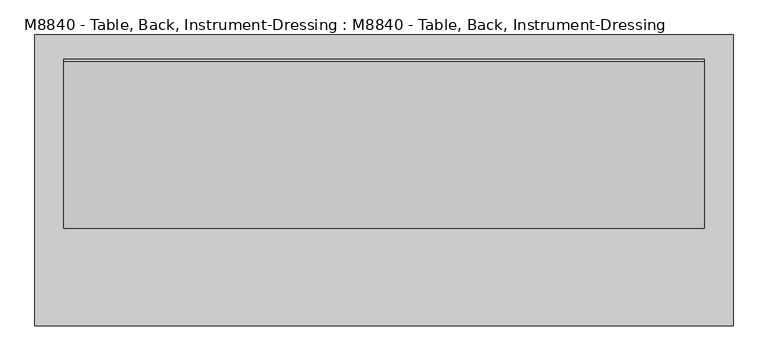
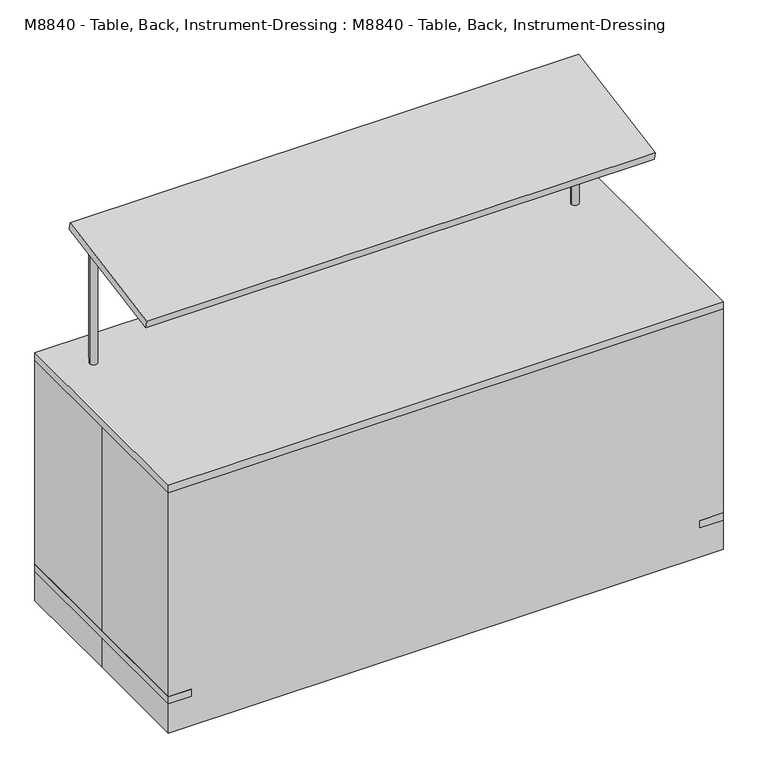
"""IFC4 building model written with IfcOpenShell, lengths in millimetres: proxy geometry, M8840 - Table, Back, Instrument-Dressing : M8840 - Table, Back, Instrument-Dressing."""

from ifc_helpers import new_model, si_unit, point, frame, frame_2d, origin, origin_with_axes, place, context, project, spatial, polyline, circle_curve, ellipse_curve, trimmed, segment, composite_curve, outline, extrude, source, transform, mapped, element, save
from ifc_brep_helpers import plane_surface, cylinder_surface, advanced_brep


def m8840_table_back_instrument_dressing_m8840_table_back_7214e6ad(model_context):
    return source(origin(), model_context, "Body", "SolidModel", [
        advanced_brep(
        [(838.2, 312.4393375, 1331.1669319), (-838.2, 312.4393375, 1331.1669319), (-838.2, -125.5940422, 1253.9298286), (838.2, -125.5940422, 1253.9298286), (838.2, 316.8500012, 1306.1528149), (838.2, -121.1833785, 1228.9157117), (-838.2, -121.1833785, 1228.9157117), (-838.2, 316.8500012, 1306.1528149), (-806.45, 255.8677573, 1295.4), (-781.05, 255.8677573, 1295.4), (806.45, 255.8677573, 1295.4), (781.05, 255.8677573, 1295.4), (-806.45, 255.8677573, 863.6), (-781.05, 255.8677573, 863.6), (806.45, 255.8677573, 863.6), (781.05, 255.8677573, 863.6)],
        [
            (0, 1),
            (1, 2),
            (2, 3),
            (3, 0),
            (4, 5),
            (5, 6),
            (6, 7),
            (7, 4),
            (8, 9, ellipse_curve(frame((-793.75, 255.8677573, 1295.4), z_axis=(0.0, -0.17364817766692925, 0.9848077530122082), x_axis=(0.0, 0.9848077530122081, 0.17364817766692942)), 12.895918, 12.7)),
            (9, 8, ellipse_curve(frame((-793.75, 255.8677573, 1295.4), z_axis=(0.0, -0.17364817766692925, 0.9848077530122082), x_axis=(0.0, 0.9848077530122081, 0.17364817766692942)), 12.895918, 12.7)),
            (10, 11, ellipse_curve(frame((793.75, 255.8677573, 1295.4), z_axis=(0.0, -0.17364817766692925, 0.9848077530122082), x_axis=(0.0, 0.9848077530122081, 0.17364817766692942)), 12.895918, 12.7)),
            (11, 10, ellipse_curve(frame((793.75, 255.8677573, 1295.4), z_axis=(0.0, -0.17364817766692925, 0.9848077530122082), x_axis=(0.0, 0.9848077530122081, 0.17364817766692942)), 12.895918, 12.7)),
            (0, 4),
            (7, 1),
            (6, 2),
            (5, 3),
            (12, 13, circle_curve(frame((-793.75, 255.8677573, 863.6), z_axis=(0.0, 0.0, -1.0), x_axis=(1.0, 0.0, 0.0)), 12.7)),
            (13, 12, circle_curve(frame((-793.75, 255.8677573, 863.6), z_axis=(0.0, 0.0, -1.0), x_axis=(1.0, 0.0, 0.0)), 12.7)),
            (14, 15, circle_curve(frame((793.75, 255.8677573, 863.6), z_axis=(0.0, 0.0, -1.0), x_axis=(-1.0, 0.0, 0.0)), 12.7)),
            (15, 14, circle_curve(frame((793.75, 255.8677573, 863.6), z_axis=(0.0, 0.0, -1.0), x_axis=(-1.0, 0.0, 0.0)), 12.7)),
            (13, 9),
            (8, 12),
            (15, 11),
            (10, 14),
        ],
        [
            plane_surface(frame((-838.2, 312.4393375, 1331.1669319), z_axis=(0.0, -0.17364817766692925, 0.9848077530122082), x_axis=(-1.0, 0.0, 0.0))),
            plane_surface(frame((-838.2, 316.8500012, 1306.1528149), z_axis=(0.0, 0.17364817766692925, -0.9848077530122082), x_axis=(1.0, 0.0, 0.0))),
            plane_surface(frame((838.2, 312.4393375, 1331.1669319), z_axis=(0.0, 0.9848077530122084, 0.17364817766692864), x_axis=(0.0, 0.17364817766692864, -0.9848077530122084))),
            plane_surface(frame((-838.2, 312.4393375, 1331.1669319), z_axis=(-1.0, 0.0, 0.0), x_axis=(0.0, 0.17364817766692864, -0.9848077530122084))),
            plane_surface(frame((-838.2, -125.5940422, 1253.9298286), z_axis=(0.0, -0.9848077530122079, -0.17364817766693125), x_axis=(0.0, 0.17364817766693125, -0.9848077530122079))),
            plane_surface(frame((838.2, -125.5940422, 1253.9298286), z_axis=(1.0, 0.0, 0.0), x_axis=(0.0, 0.17364817766692864, -0.9848077530122084))),
            plane_surface(frame((-781.05, 255.8677573, 863.6), z_axis=(0.0, 0.0, -1.0), x_axis=(0.0, -1.0, 0.0))),
            cylinder_surface(frame((-793.75, 255.8677573, 863.6), z_axis=(0.0, 0.0, 1.0), x_axis=(1.0, 0.0, 0.0)), 12.7),
            cylinder_surface(frame((793.75, 255.8677573, 0.0), z_axis=(0.0, 0.0, 1.0), x_axis=(-1.0, 0.0, 0.0)), 12.7),
        ],
        [
            (0, [[1, 2, 3, 4]]),
            (1, [[5, 6, 7, 8], [9, 10], [11, 12]]),
            (2, [[-1, 13, -8, 14]]),
            (3, [[-2, -14, -7, 15]]),
            (4, [[-3, -15, -6, 16]]),
            (5, [[-4, -16, -5, -13]]),
            (6, [[17, 18]]),
            (6, [[19, 20]]),
            (7, [[-18, 21, -9, 22]]),
            (7, [[-17, -22, -10, -21]]),
            (8, [[-20, 23, -11, 24]]),
            (8, [[-19, -24, -12, -23]]),
        ],
    ),
        extrude(outline(polyline([(869.95, 290.561646), (863.6, 290.561646), (863.6, 317.7907506), (869.95, 317.7907506), (869.95, 290.561646)])), frame((0.0, 0.0, 50.8), z_axis=(0.0, 0.0, 1.0), x_axis=(1.0, 0.0, 0.0)), (0.0, 0.0, 1.0), 50.8),
        extrude(outline(polyline([(889.0, 290.561646), (882.65, 290.561646), (882.65, 317.7907506), (889.0, 317.7907506), (889.0, 290.561646)])), frame((0.0, 0.0, 50.8), z_axis=(0.0, 0.0, 1.0), x_axis=(1.0, 0.0, 0.0)), (0.0, 0.0, 1.0), 50.8),
        extrude(outline(composite_curve([segment(trimmed(circle_curve(frame_2d((304.8, 50.8)), 50.8), [point((355.6, 50.8))], [point((254.0, 50.8))], False, "CARTESIAN"), True, "CONTINUOUS"), segment(trimmed(circle_curve(frame_2d((304.8, 50.8)), 50.8), [point((254.0, 50.8))], [point((355.6, 50.8))], False, "CARTESIAN"), True, "CONTINUOUS")], self_intersect=False)), frame((869.95, 0.0, 0.0), z_axis=(1.0, 0.0, 0.0), x_axis=(0.0, 1.0, 0.0)), (0.0, 0.0, 1.0), 12.7),
        extrude(outline(polyline([(-882.65, 290.561646), (-889.0, 290.561646), (-889.0, 317.7907506), (-882.65, 317.7907506), (-882.65, 290.561646)])), frame((0.0, 0.0, 50.8), z_axis=(0.0, 0.0, 1.0), x_axis=(1.0, 0.0, 0.0)), (0.0, 0.0, 1.0), 50.8),
        extrude(outline(polyline([(-863.6, 290.561646), (-869.95, 290.561646), (-869.95, 317.7907506), (-863.6, 317.7907506), (-863.6, 290.561646)])), frame((0.0, 0.0, 50.8), z_axis=(0.0, 0.0, 1.0), x_axis=(1.0, 0.0, 0.0)), (0.0, 0.0, 1.0), 50.8),
        extrude(outline(composite_curve([segment(trimmed(circle_curve(frame_2d((304.8, 50.8)), 50.8), [point((355.6, 50.8))], [point((254.0, 50.8))], False, "CARTESIAN"), True, "CONTINUOUS"), segment(trimmed(circle_curve(frame_2d((304.8, 50.8)), 50.8), [point((254.0, 50.8))], [point((355.6, 50.8))], False, "CARTESIAN"), True, "CONTINUOUS")], self_intersect=False)), frame((-882.65, 0.0, 0.0), z_axis=(1.0, 0.0, 0.0), x_axis=(0.0, 1.0, 0.0)), (0.0, 0.0, 1.0), 12.7),
        extrude(outline(polyline([(869.95, -319.038354), (863.6, -319.038354), (863.6, -291.8092494), (869.95, -291.8092494), (869.95, -319.038354)])), frame((0.0, 0.0, 50.8), z_axis=(0.0, 0.0, 1.0), x_axis=(1.0, 0.0, 0.0)), (0.0, 0.0, 1.0), 50.8),
        extrude(outline(polyline([(889.0, -319.038354), (882.65, -319.038354), (882.65, -291.8092494), (889.0, -291.8092494), (889.0, -319.038354)])), frame((0.0, 0.0, 50.8), z_axis=(0.0, 0.0, 1.0), x_axis=(1.0, 0.0, 0.0)), (0.0, 0.0, 1.0), 50.8),
        extrude(outline(composite_curve([segment(trimmed(circle_curve(frame_2d((-304.8, 50.8)), 50.8), [point((-254.0, 50.8))], [point((-355.6, 50.8))], False, "CARTESIAN"), True, "CONTINUOUS"), segment(trimmed(circle_curve(frame_2d((-304.8, 50.8)), 50.8), [point((-355.6, 50.8))], [point((-254.0, 50.8))], False, "CARTESIAN"), True, "CONTINUOUS")], self_intersect=False)), frame((869.95, 0.0, 0.0), z_axis=(1.0, 0.0, 0.0), x_axis=(0.0, 1.0, 0.0)), (0.0, 0.0, 1.0), 12.7),
        extrude(outline(polyline([(-882.65, -319.038354), (-889.0, -319.038354), (-889.0, -291.8092494), (-882.65, -291.8092494), (-882.65, -319.038354)])), frame((0.0, 0.0, 50.8), z_axis=(0.0, 0.0, 1.0), x_axis=(1.0, 0.0, 0.0)), (0.0, 0.0, 1.0), 50.8),
        extrude(outline(polyline([(-863.6, -319.038354), (-869.95, -319.038354), (-869.95, -291.8092494), (-863.6, -291.8092494), (-863.6, -319.038354)])), frame((0.0, 0.0, 50.8), z_axis=(0.0, 0.0, 1.0), x_axis=(1.0, 0.0, 0.0)), (0.0, 0.0, 1.0), 50.8),
        extrude(outline(composite_curve([segment(trimmed(circle_curve(frame_2d((-304.8, 50.8)), 50.8), [point((-254.0, 50.8))], [point((-355.6, 50.8))], False, "CARTESIAN"), True, "CONTINUOUS"), segment(trimmed(circle_curve(frame_2d((-304.8, 50.8)), 50.8), [point((-355.6, 50.8))], [point((-254.0, 50.8))], False, "CARTESIAN"), True, "CONTINUOUS")], self_intersect=False)), frame((-882.65, 0.0, 0.0), z_axis=(1.0, 0.0, 0.0), x_axis=(0.0, 1.0, 0.0)), (0.0, 0.0, 1.0), 12.7),
        extrude(outline(polyline([(914.4, 381.0), (914.4, -381.0), (-914.4, -381.0), (-914.4, 381.0), (914.4, 381.0)])), frame((0.0, 0.0, 838.2), z_axis=(0.0, 0.0, 1.0), x_axis=(1.0, 0.0, 0.0)), (0.0, 0.0, 1.0), 25.4),
        extrude(outline(composite_curve([segment(trimmed(circle_curve(frame_2d((876.3, -304.8)), 25.4), [point((876.3, -279.4))], [point((850.9, -304.8))], True, "CARTESIAN"), True, "CONTINUOUS"), segment(polyline([(850.9, -304.8), (-850.9, -304.8)]), True, "CONTINUOUS"), segment(trimmed(circle_curve(frame_2d((-876.3, -304.8)), 25.4), [point((-850.9, -304.8))], [point((-876.3, -279.4))], True, "CARTESIAN"), True, "CONTINUOUS"), segment(polyline([(-876.3, -279.4), (-876.3, 279.4)]), True, "CONTINUOUS"), segment(trimmed(circle_curve(frame_2d((-876.3, 304.8)), 25.4), [point((-876.3, 279.4))], [point((-850.9, 304.8))], True, "CARTESIAN"), True, "CONTINUOUS"), segment(polyline([(-850.9, 304.8), (850.9, 304.8)]), True, "CONTINUOUS"), segment(trimmed(circle_curve(frame_2d((876.3, 304.8)), 25.4), [point((850.9, 304.8))], [point((876.3, 279.4))], True, "CARTESIAN"), True, "CONTINUOUS"), segment(polyline([(876.3, 279.4), (876.3, -279.4)]), True, "CONTINUOUS")], self_intersect=False)), frame((0.0, 0.0, 279.4), z_axis=(0.0, 0.0, 1.0), x_axis=(1.0, 0.0, 0.0)), (0.0, 0.0, 1.0), 25.4),
        extrude(outline(composite_curve([segment(trimmed(circle_curve(frame_2d((-876.3, -304.8)), 25.4), [point((-901.7, -304.8))], [point((-850.9, -304.8))], False, "CARTESIAN"), True, "CONTINUOUS"), segment(trimmed(circle_curve(frame_2d((-876.3, -304.8)), 25.4), [point((-850.9, -304.8))], [point((-901.7, -304.8))], False, "CARTESIAN"), True, "CONTINUOUS")], self_intersect=False)), frame((0.0, 0.0, 127.0), z_axis=(0.0, 0.0, 1.0), x_axis=(1.0, 0.0, 0.0)), (0.0, 0.0, 1.0), 711.2),
        extrude(outline(composite_curve([segment(trimmed(circle_curve(frame_2d((876.3, -304.8)), 25.4), [point((901.7, -304.8))], [point((850.9, -304.8))], False, "CARTESIAN"), True, "CONTINUOUS"), segment(trimmed(circle_curve(frame_2d((876.3, -304.8)), 25.4), [point((850.9, -304.8))], [point((901.7, -304.8))], False, "CARTESIAN"), True, "CONTINUOUS")], self_intersect=False)), frame((0.0, 0.0, 127.0), z_axis=(0.0, 0.0, 1.0), x_axis=(1.0, 0.0, 0.0)), (0.0, 0.0, 1.0), 711.2),
        extrude(outline(composite_curve([segment(trimmed(circle_curve(frame_2d((-876.3, 304.8)), 25.4), [point((-901.7, 304.8))], [point((-850.9, 304.8))], False, "CARTESIAN"), True, "CONTINUOUS"), segment(trimmed(circle_curve(frame_2d((-876.3, 304.8)), 25.4), [point((-850.9, 304.8))], [point((-901.7, 304.8))], False, "CARTESIAN"), True, "CONTINUOUS")], self_intersect=False)), frame((0.0, 0.0, 127.0), z_axis=(0.0, 0.0, 1.0), x_axis=(1.0, 0.0, 0.0)), (0.0, 0.0, 1.0), 711.2),
        extrude(outline(composite_curve([segment(trimmed(circle_curve(frame_2d((876.3, 304.8)), 25.4), [point((901.7, 304.8))], [point((850.9, 304.8))], False, "CARTESIAN"), True, "CONTINUOUS"), segment(trimmed(circle_curve(frame_2d((876.3, 304.8)), 25.4), [point((850.9, 304.8))], [point((901.7, 304.8))], False, "CARTESIAN"), True, "CONTINUOUS")], self_intersect=False)), frame((0.0, 0.0, 127.0), z_axis=(0.0, 0.0, 1.0), x_axis=(1.0, 0.0, 0.0)), (0.0, 0.0, 1.0), 711.2),
        extrude(outline(polyline([(-838.2, 381.0), (-838.2, -381.0), (-914.4, -381.0), (-914.4, 381.0), (-838.2, 381.0)])), frame((0.0, 0.0, 101.6), z_axis=(0.0, 0.0, 1.0), x_axis=(1.0, 0.0, 0.0)), (0.0, 0.0, 1.0), 25.4),
        extrude(outline(polyline([(838.2, 381.0), (914.4, 381.0), (914.4, -381.0), (838.2, -381.0), (838.2, 381.0)])), frame((0.0, 0.0, 101.6), z_axis=(0.0, 0.0, 1.0), x_axis=(1.0, 0.0, 0.0)), (0.0, 0.0, 1.0), 25.4),
        extrude(outline(polyline([(-914.4, 381.0), (914.4, 381.0), (914.4, -381.0), (-914.4, -381.0), (-914.4, 0.0), (-914.4, 381.0)])), origin_with_axes(), (0.0, 0.0, 1.0), 863.6),
    ])


if __name__ == "__main__":
    model = new_model("IFC4")
    model_context = context("Model", 3, world=origin())
    ifc_project = project(units=[si_unit("LENGTHUNIT", "METRE", prefix="MILLI")], contexts=[model_context])
    site = spatial("IfcSite", under=ifc_project)
    building = spatial("IfcBuilding", under=site)
    placement = place(None, origin())
    m8840_table_back_instrument_dressing_m8840_table_back_shape = m8840_table_back_instrument_dressing_m8840_table_back_7214e6ad(model_context)
    element("IfcBuildingElementProxy", 1, Name="M8840 - Table, Back, Instrument-Dressing : M8840 - Table, Back, Instrument-Dressing", ObjectType="M8840 - Table, Back, Instrument-Dressing : M8840 - Table, Back, Instrument-Dressing", at=placement, inside=building, context=model_context, shape_type="MappedRepresentation", body=[
        mapped(m8840_table_back_instrument_dressing_m8840_table_back_shape, transform((0.0, 0.0, 0.0), x_axis=(1.0, 0.0, 0.0), y_axis=(0.0, 1.0, 0.0), z_axis=(0.0, 0.0, 1.0))),
    ])
    save(model, "model.ifc")

# Revit data of these elements
# Type "M8840 - Table, Back, Instrument-Dressing : M8840 - Table, Back, Instrument-Dressing"
#   JSN = "M8840"
#   Nomenclature = "Table, Back, Instrument/Dressing"
#   UTIL_1_WaterDrain = "-"
#   UTIL_2_Elec = "-"
#   UTIL_3_MedGas = "-"
#   UTIL_4_MiscGas = "-"
#   UTIL_5_NonMedGas = "-"
#   UTIL_6_Misc = "-"
#   Utility_6 = "-"
#   Utility_5 = "-"
#   Utility_4 = "-"
#   Utility_3 = "-"
#   Utility_2 = "-"
#   Utility_1 = "-"
#   Unit_Issue = "EA"
#   Price_Date = "02/05/2014"
#   Nomenclature = "Table, Back, Instrument/Dressing"
#   NSN = "6515"
#   Location [instance default] = ""
#   JSN_Name = "M8840"
#   Hertz_swit = "0"
#   Hertz_dep = "0"
#   Hertz = "0"
#   Desc = "A specialty back table for large cases such as orthopedics, spinal fusions, neuro and craniotomies. The table has a pneumatic tuck-away cantilevered shelf which can hold multiple trays and is angled for clear observation of instruments. It comes with 4\" diameter heavy-duty ball bearing brake/swivel casters. Construction is all stainless steel."
#   CAT_VA = "-"
#   CAT_Navy = "C"
#   CAT_IHS = "C"
#   CAT_Army = "C"
#   CAT_AF = "-"
#   BTUPerHour = "0"
#   Width_IN = 72
#   Weight_AV = 0
#   Watts2 = 0
#   Watts1 = 0
#   Volts2 = 0
#   Volts1 = 0
#   Phase2 = 0
#   Phase1 = 0
#   Height_IN = 34
#   Depth_IN = 30
#   Amps2 = 0
#   Amps1 = 0
# Element 1 (IfcBuildingElementProxy, "M8840 - Table, Back, Instrument-Dressing : M8840 - Table, Back, Instrument-Dressing")
#   Materials on its faces: "EquipSpace"
# Materials
#   "EquipSpace": class "Unassigned", colour RGB 221 217 195, transparency 0.5
